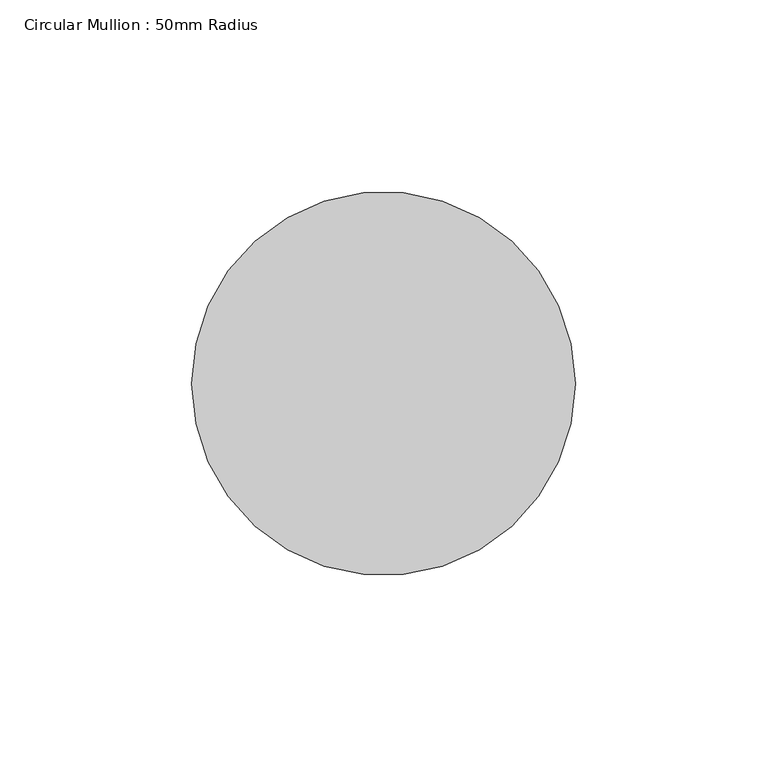
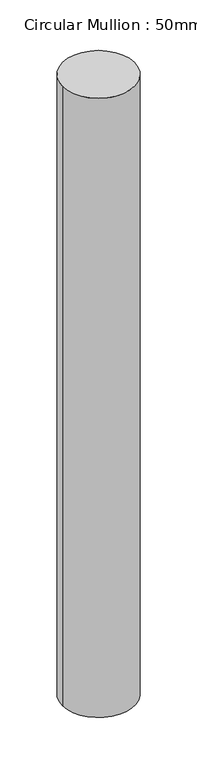
"""IFC4 building model written with IfcOpenShell, lengths in millimetres: member geometry, Circular Mullion : 50mm Radius."""

from ifc_helpers import new_model, si_unit, point, frame, origin, origin_2d, place, context, project, spatial, circle_curve, trimmed, segment, composite_curve, outline, extrude, source, transform, mapped, element, save


def circular_mullion_50mm_radius_9faaf5eb(model_context):
    return source(origin(), model_context, "Body", "SweptSolid", [
        extrude(outline(composite_curve([segment(trimmed(circle_curve(origin_2d(), 50.0), [point((50.0, 0.0))], [point((-50.0, 0.0))], False, "CARTESIAN"), True, "CONTINUOUS"), segment(trimmed(circle_curve(origin_2d(), 50.0), [point((-50.0, 0.0))], [point((50.0, 0.0))], False, "CARTESIAN"), True, "CONTINUOUS")], self_intersect=False)), frame((0.0, 0.0, -905.9304336), z_axis=(0.0, 0.0, 1.0), x_axis=(1.0, 0.0, 0.0)), (0.0, 0.0, 1.0), 905.9304336),
    ])


if __name__ == "__main__":
    model = new_model("IFC4")
    model_context = context("Model", 3, world=origin())
    ifc_project = project(units=[si_unit("LENGTHUNIT", "METRE", prefix="MILLI")], contexts=[model_context])
    site = spatial("IfcSite", under=ifc_project)
    building = spatial("IfcBuilding", under=site)
    placement = place(None, origin())
    circular_mullion_50mm_radius_shape = circular_mullion_50mm_radius_9faaf5eb(model_context)
    element("IfcMember", 1, ObjectType="Circular Mullion : 50mm Radius", at=placement, inside=building, context=model_context, shape_type="MappedRepresentation", body=[
        mapped(circular_mullion_50mm_radius_shape, transform((0.0, 0.0, 0.0), x_axis=(1.0, 0.0, 0.0), y_axis=(0.0, 1.0, 0.0), z_axis=(0.0, 0.0, 1.0))),
    ])
    save(model, "model.ifc")

# Revit data of these elements
# Type "Circular Mullion : 50mm Radius"
#   built-in parameter 1007350 = 0.164042 (stored number, unit not read)
# Element 1 (IfcMember, "Circular Mullion : 50mm Radius")
#   Materials on its faces: "Aluminium"
# Materials
#   "Aluminium": class "Metal", colour RGB 247 247 247, transparency 0, Description = "Aluminium 6061", Cost = 0
